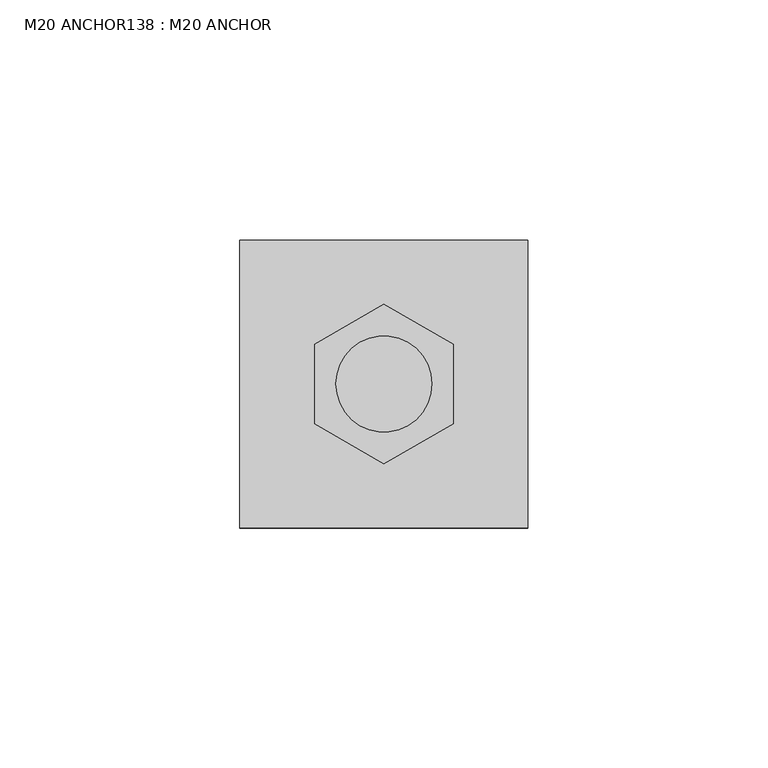
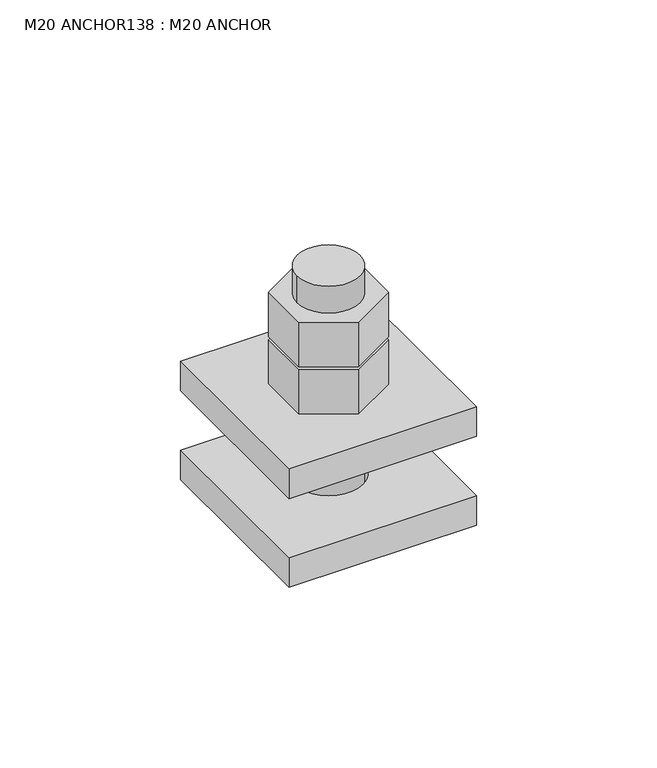
"""IFC4 building model written with IfcOpenShell, lengths in millimetres: fastener geometry, M20 ANCHOR138 : M20 ANCHOR."""

from ifc_helpers import new_model, si_unit, point, frame, frame_2d, origin, place, context, project, spatial, polyline, circle_curve, trimmed, segment, composite_curve, outline, extrude, source, transform, mapped, element, save


def m20_anchor138_m20_anchor_b4f80572(model_context):
    return source(origin(), model_context, "Body", "SweptSolid", [
        extrude(outline(polyline([(5991.9144032, 22453.9464399), (5977.5062842, 22445.6279085), (5963.0981652, 22453.9464399), (5963.0981652, 22470.5835027), (5977.5062842, 22478.9020341), (5991.9144032, 22470.5835027), (5991.9144032, 22453.9464399)]), holes=[composite_curve([segment(trimmed(circle_curve(frame_2d((5977.5062842, 22462.2649713)), 10.0), [point((5967.5062842, 22462.2649713))], [point((5987.5062842, 22462.2649713))], True, "CARTESIAN"), True, "CONTINUOUS"), segment(trimmed(circle_curve(frame_2d((5977.5062842, 22462.2649713)), 10.0), [point((5987.5062842, 22462.2649713))], [point((5967.5062842, 22462.2649713))], True, "CARTESIAN"), True, "CONTINUOUS")], self_intersect=False)]), frame((0.0, 0.0, 246.0), z_axis=(0.0, 0.0, 1.0), x_axis=(1.0, 0.0, 0.0)), (0.0, 0.0, 1.0), 15.0),
        extrude(outline(polyline([(5991.9144032, 22453.9464399), (5977.5062842, 22445.6279085), (5963.0981652, 22453.9464399), (5963.0981652, 22470.5835027), (5977.5062842, 22478.9020341), (5991.9144032, 22470.5835027), (5991.9144032, 22453.9464399)]), holes=[composite_curve([segment(trimmed(circle_curve(frame_2d((5977.5062842, 22462.2649713)), 10.0), [point((5967.5062842, 22462.2649713))], [point((5987.5062842, 22462.2649713))], True, "CARTESIAN"), True, "CONTINUOUS"), segment(trimmed(circle_curve(frame_2d((5977.5062842, 22462.2649713)), 10.0), [point((5987.5062842, 22462.2649713))], [point((5967.5062842, 22462.2649713))], True, "CARTESIAN"), True, "CONTINUOUS")], self_intersect=False)]), frame((0.0, 0.0, 230.0), z_axis=(0.0, 0.0, 1.0), x_axis=(1.0, 0.0, 0.0)), (0.0, 0.0, 1.0), 15.0),
        extrude(outline(composite_curve([segment(trimmed(circle_curve(frame_2d((5977.5062842, 22462.2649713)), 10.0), [point((5967.5062842, 22462.2649713))], [point((5987.5062842, 22462.2649713))], False, "CARTESIAN"), True, "CONTINUOUS"), segment(trimmed(circle_curve(frame_2d((5977.5062842, 22462.2649713)), 10.0), [point((5987.5062842, 22462.2649713))], [point((5967.5062842, 22462.2649713))], False, "CARTESIAN"), True, "CONTINUOUS")], self_intersect=False)), frame((0.0, 0.0, 190.0), z_axis=(0.0, 0.0, 1.0), x_axis=(1.0, 0.0, 0.0)), (0.0, 0.0, 1.0), 80.0),
        extrude(outline(polyline([(6007.5062842, 22432.2649713), (5947.5062842, 22432.2649713), (5947.5062842, 22492.2649713), (6007.5062842, 22492.2649713), (6007.5062842, 22432.2649713)]), holes=[composite_curve([segment(trimmed(circle_curve(frame_2d((5977.5062842, 22462.2649713)), 11.0), [point((5966.5062842, 22462.2649713))], [point((5988.5062842, 22462.2649713))], True, "CARTESIAN"), True, "CONTINUOUS"), segment(trimmed(circle_curve(frame_2d((5977.5062842, 22462.2649713)), 11.0), [point((5988.5062842, 22462.2649713))], [point((5966.5062842, 22462.2649713))], True, "CARTESIAN"), True, "CONTINUOUS")], self_intersect=False)]), frame((0.0, 0.0, 190.0), z_axis=(0.0, 0.0, 1.0), x_axis=(1.0, 0.0, 0.0)), (0.0, 0.0, 1.0), 10.0),
        extrude(outline(polyline([(6007.5062842, 22432.2649713), (5947.5062842, 22432.2649713), (5947.5062842, 22492.2649713), (6007.5062842, 22492.2649713), (6007.5062842, 22432.2649713)]), holes=[composite_curve([segment(trimmed(circle_curve(frame_2d((5977.5062842, 22462.2649713)), 11.0), [point((5966.5062842, 22462.2649713))], [point((5988.5062842, 22462.2649713))], True, "CARTESIAN"), True, "CONTINUOUS"), segment(trimmed(circle_curve(frame_2d((5977.5062842, 22462.2649713)), 11.0), [point((5988.5062842, 22462.2649713))], [point((5966.5062842, 22462.2649713))], True, "CARTESIAN"), True, "CONTINUOUS")], self_intersect=False)]), frame((0.0, 0.0, 220.0), z_axis=(0.0, 0.0, 1.0), x_axis=(1.0, 0.0, 0.0)), (0.0, 0.0, 1.0), 10.0),
    ])


if __name__ == "__main__":
    model = new_model("IFC4")
    model_context = context("Model", 3, world=origin())
    ifc_project = project(units=[si_unit("LENGTHUNIT", "METRE", prefix="MILLI")], contexts=[model_context])
    site = spatial("IfcSite", under=ifc_project)
    building = spatial("IfcBuilding", under=site)
    placement = place(None, origin())
    m20_anchor138_m20_anchor_shape = m20_anchor138_m20_anchor_b4f80572(model_context)
    element("IfcFastener", 1, ObjectType="M20 ANCHOR138 : M20 ANCHOR", at=placement, inside=building, context=model_context, shape_type="MappedRepresentation", body=[
        mapped(m20_anchor138_m20_anchor_shape, transform((0.0, 0.0, 0.0), x_axis=(1.0, 0.0, 0.0), y_axis=(0.0, 1.0, 0.0), z_axis=(0.0, 0.0, 1.0))),
    ])
    save(model, "model.ifc")
